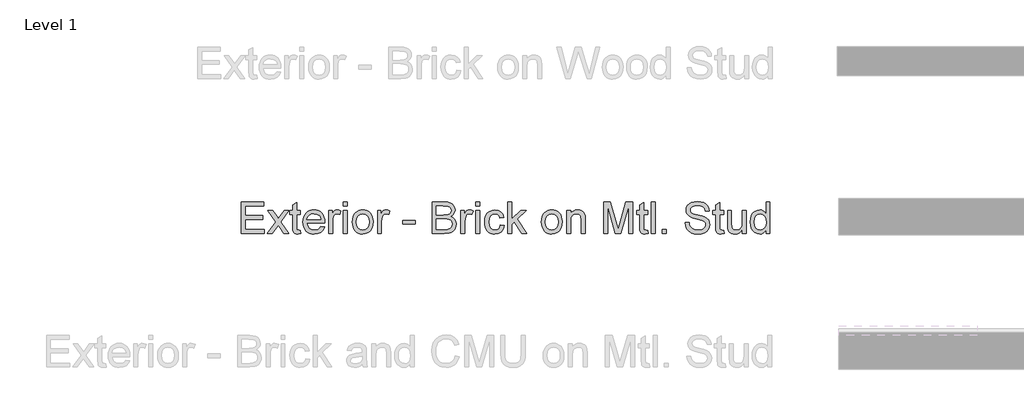
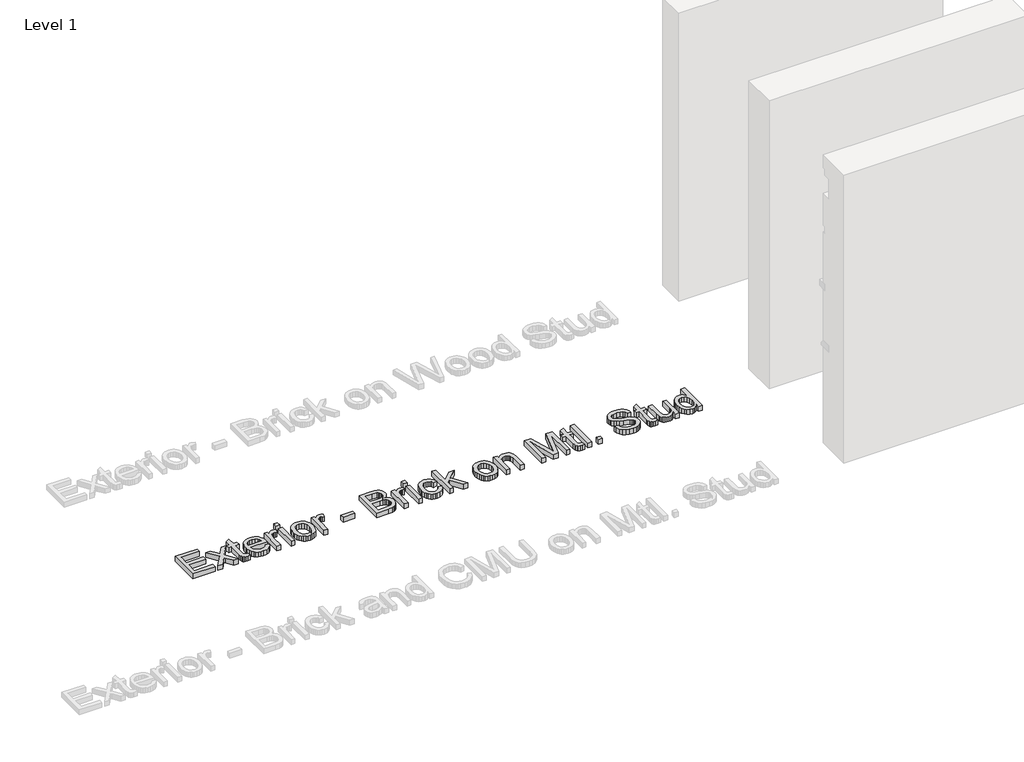
# One storey, part 27 of 42: 1 proxy.
"""IFC4 building model written with IfcOpenShell, lengths in millimetres."""

from ifc_helpers import new_model, si_unit, origin, origin_with_axes, place, context, project, spatial, polyline, outline, extrude, element, save

model = new_model("IFC4")

# Units and contexts
model_context = context("Model", 3, world=origin())
ifc_project = project(units=[si_unit("LENGTHUNIT", "METRE", prefix="MILLI")], contexts=[model_context])

# Site, building, storey
site = spatial("IfcSite", under=ifc_project)
building = spatial("IfcBuilding", under=site)
storey = spatial("IfcBuildingStorey", under=building, Name="Level 1", Elevation=0.0)

# Proxy
placement = place(None, origin())
element("IfcBuildingElementProxy", 1, Name="8\" Arial", ObjectType="8\" Arial", at=placement, inside=storey, context=model_context, shape_type="SweptSolid", body=[
    extrude(outline(polyline([(-5074.4671902, 11235.919571), (-5074.4671902, 11540.4866651), (-4855.5595914, 11540.4866651), (-4855.5595914, 11502.4157783), (-5036.3963035, 11502.4157783), (-5036.3963035, 11411.9974223), (-4865.0773131, 11411.9974223), (-4865.0773131, 11373.9265355), (-5036.3963035, 11373.9265355), (-5036.3963035, 11273.9904578), (-4850.8007305, 11273.9904578), (-4850.8007305, 11235.919571), (-5074.4671902, 11235.919571)])), origin_with_axes(), (0.0, 0.0, 1.0), 50.8),
    extrude(outline(polyline([(-4822.2475655, 11235.919571), (-4740.9007879, 11348.3476585), (-4817.4887046, 11459.5860307), (-4771.684669, 11459.5860307), (-4734.7291402, 11406.0488462), (-4717.4782697, 11380.767398), (-4702.5324723, 11401.4386998), (-4660.4462967, 11459.5860307), (-4614.6422611, 11459.5860307), (-4695.0967523, 11348.3476585), (-4617.6165491, 11235.919571), (-4663.4205848, 11235.919571), (-4710.0425496, 11303.5102665), (-4718.5936277, 11315.8535618), (-4776.4435298, 11235.919571), (-4822.2475655, 11235.919571)])), origin_with_axes(), (0.0, 0.0, 1.0), 50.8),
    extrude(outline(polyline([(-4503.4038889, 11267.6700957), (-4498.645028, 11234.804213), (-4527.1238359, 11231.1607102), (-4545.397118, 11232.7408007), (-4559.023075, 11237.4810723), (-4568.6523325, 11244.7866672), (-4574.9355159, 11254.062728), (-4578.3931258, 11269.9937583), (-4579.5456624, 11297.2642616), (-4579.5456624, 11421.515144), (-4608.0988274, 11421.515144), (-4608.0988274, 11459.5860307), (-4579.5456624, 11459.5860307), (-4579.5456624, 11513.9411445), (-4541.4747756, 11536.3226619), (-4541.4747756, 11459.5860307), (-4503.4038889, 11459.5860307), (-4503.4038889, 11421.515144), (-4541.4747756, 11421.515144), (-4541.4747756, 11298.3796196), (-4539.4671312, 11278.7493186), (-4532.9608761, 11271.7969204), (-4519.9855446, 11269.231597), (-4503.4038889, 11267.6700957)])), origin_with_axes(), (0.0, 0.0, 1.0), 50.8),
    extrude(outline(polyline([(-4308.7367374, 11302.5436229), (-4271.4094227, 11297.784762), (-4284.8587814, 11269.6591509), (-4306.3201284, 11248.6346524), (-4335.310142, 11235.5291957), (-4371.3455004, 11231.1607102), (-4394.9678536, 11233.0452005), (-4416.0155887, 11238.6986714), (-4434.4887058, 11248.1211229), (-4450.3872048, 11261.3125551), (-4463.171996, 11277.9058291), (-4472.3039897, 11297.5338065), (-4477.7831859, 11320.196487), (-4479.6095846, 11345.8938709), (-4477.7645966, 11372.4626281), (-4472.2296325, 11395.880499), (-4463.0046923, 11416.1474836), (-4450.089776, 11433.2635817), (-4434.2331029, 11446.8616548), (-4416.1828924, 11456.5745641), (-4395.9391445, 11462.4023097), (-4373.5018592, 11464.3448916), (-4351.787233, 11462.406957), (-4332.149961, 11456.5931534), (-4314.5900433, 11446.9034807), (-4299.1074799, 11433.3379389), (-4286.4690795, 11416.2590194), (-4277.4416506, 11396.0292134), (-4272.0251932, 11372.6485212), (-4270.2197075, 11346.1169425), (-4270.4427791, 11335.8556488), (-4441.5386979, 11335.8556488), (-4434.948791, 11307.3582516), (-4419.6405023, 11286.4081103), (-4397.547119, 11273.5257253), (-4370.6019284, 11269.231597), (-4350.3395912, 11271.2206521), (-4333.2746137, 11277.1878174), (-4319.4069957, 11287.504879), (-4308.7367374, 11302.5436229)]), holes=[polyline([(-4441.5386979, 11373.9265355), (-4308.2905942, 11373.9265355), (-4313.4398304, 11394.0401583), (-4323.5338204, 11408.4282767), (-4345.7294448, 11421.8125728), (-4373.6505736, 11426.2740048), (-4399.3131025, 11422.7141538), (-4420.5327887, 11412.0346009), (-4435.2833984, 11395.3878826), (-4441.5386979, 11373.9265355)])]), origin_with_axes(), (0.0, 0.0, 1.0), 50.8),
    extrude(outline(polyline([(-4232.1488207, 11235.919571), (-4232.1488207, 11459.5860307), (-4198.8367948, 11459.5860307), (-4198.8367948, 11426.4970764), (-4186.5306781, 11445.6812342), (-4175.191205, 11456.9835287), (-4163.8145533, 11462.5045509), (-4151.3969007, 11464.3448916), (-4132.4358146, 11461.4077822), (-4113.1772996, 11452.5964539), (-4125.8923809, 11418.4664988), (-4139.276677, 11424.3221283), (-4152.6609732, 11426.2740048), (-4164.0283302, 11424.3964855), (-4174.1873828, 11418.7639276), (-4182.3945588, 11409.8038849), (-4187.9062863, 11397.9439114), (-4192.535022, 11376.677752), (-4194.0779339, 11353.4783053), (-4194.0779339, 11235.919571), (-4232.1488207, 11235.919571)])), origin_with_axes(), (0.0, 0.0, 1.0), 50.8),
    extrude(outline(polyline([(-4089.3829954, 11502.4157783), (-4089.3829954, 11540.4866651), (-4051.3121086, 11540.4866651), (-4051.3121086, 11502.4157783), (-4089.3829954, 11502.4157783)])), origin_with_axes(), (0.0, 0.0, 1.0), 50.8),
    extrude(outline(polyline([(-4089.3829954, 11235.919571), (-4089.3829954, 11459.5860307), (-4051.3121086, 11459.5860307), (-4051.3121086, 11235.919571), (-4089.3829954, 11235.919571)])), origin_with_axes(), (0.0, 0.0, 1.0), 50.8),
    extrude(outline(polyline([(-4003.7235002, 11347.7528009), (-4001.6647352, 11376.7195779), (-3995.4884402, 11401.6803607), (-3985.1946152, 11422.6351493), (-3970.7832602, 11439.5839438), (-3956.2743115, 11450.4168584), (-3940.2596294, 11458.1546546), (-3922.7392139, 11462.7973323), (-3903.7130652, 11464.3448916), (-3882.7094797, 11462.4604013), (-3863.7181859, 11456.8069304), (-3846.7391838, 11447.3844788), (-3831.7724735, 11434.1930467), (-3819.5569797, 11417.6787772), (-3810.8316269, 11398.2878134), (-3805.5964152, 11376.0201555), (-3803.8513447, 11350.8758033), (-3806.9371685, 11312.4145413), (-3816.19464, 11283.1363935), (-3831.3542143, 11261.2103139), (-3852.1463465, 11244.8052565), (-3876.8422318, 11234.5718468), (-3903.7130652, 11231.1607102), (-3925.0233742, 11233.0382295), (-3944.1912663, 11238.6707875), (-3961.2167416, 11248.0583841), (-3976.0998001, 11261.2010193), (-3988.1851689, 11277.8756215), (-3996.8175751, 11297.8591192), (-4001.9970189, 11321.1515123), (-4003.7235002, 11347.7528009)]), holes=[polyline([(-3965.6526134, 11347.8271581), (-3961.2469493, 11313.3718902), (-3948.0299568, 11288.8247193), (-3928.1394056, 11274.1298775), (-3903.7130652, 11269.231597), (-3879.3982606, 11274.1577615), (-3859.544888, 11288.9362551), (-3846.3278956, 11313.8087388), (-3841.9222314, 11349.0168733), (-3846.3557795, 11382.468319), (-3859.6564238, 11406.6808824), (-3879.5376803, 11421.3757242), (-3903.7130652, 11426.2740048), (-3928.1394056, 11421.3943135), (-3948.0299568, 11406.7552396), (-3961.2469493, 11382.2638367), (-3965.6526134, 11347.8271581)])]), origin_with_axes(), (0.0, 0.0, 1.0), 50.8),
    extrude(outline(polyline([(-3761.0215971, 11235.919571), (-3761.0215971, 11459.5860307), (-3727.7095712, 11459.5860307), (-3727.7095712, 11426.4970764), (-3715.4034544, 11445.6812342), (-3704.0639813, 11456.9835287), (-3692.6873296, 11462.5045509), (-3680.2696771, 11464.3448916), (-3661.3085909, 11461.4077822), (-3642.0500759, 11452.5964539), (-3654.7651573, 11418.4664988), (-3668.1494534, 11424.3221283), (-3681.5337495, 11426.2740048), (-3692.9011066, 11424.3964855), (-3703.0601591, 11418.7639276), (-3711.2673352, 11409.8038849), (-3716.7790627, 11397.9439114), (-3721.4077984, 11376.677752), (-3722.9507103, 11353.4783053), (-3722.9507103, 11235.919571), (-3761.0215971, 11235.919571)])), origin_with_axes(), (0.0, 0.0, 1.0), 50.8),
    extrude(outline(polyline([(-3518.319694, 11326.3379271), (-3518.319694, 11364.4088138), (-3399.3481729, 11364.4088138), (-3399.3481729, 11326.3379271), (-3518.319694, 11326.3379271)])), origin_with_axes(), (0.0, 0.0, 1.0), 50.8),
    extrude(outline(polyline([(-3232.7880433, 11235.919571), (-3232.7880433, 11540.4866651), (-3116.5677386, 11540.4866651), (-3084.6034369, 11538.2466544), (-3059.6473015, 11531.5266224), (-3040.5189116, 11520.1592654), (-3026.0378467, 11503.9772796), (-3016.919795, 11484.9418362), (-3013.8804444, 11465.0141064), (-3016.4364732, 11446.6757618), (-3024.1045595, 11429.4341859), (-3036.9404713, 11414.3489688), (-3054.9999764, 11402.4797006), (-3033.4270936, 11391.2145847), (-3017.4867687, 11374.0752499), (-3007.6437342, 11352.1956436), (-3004.3627227, 11326.7097131), (-3006.6027334, 11305.4714376), (-3013.3227654, 11285.7760741), (-3023.3516929, 11269.0271146), (-3035.5183898, 11256.6280514), (-3050.4177139, 11247.6494194), (-3068.6445227, 11241.1617537), (-3117.460025, 11235.919571), (-3232.7880433, 11235.919571)]), holes=[polyline([(-3194.7171565, 11416.7562831), (-3125.1931739, 11416.7562831), (-3084.5941423, 11420.028), (-3070.3826223, 11425.6698526), (-3060.1678019, 11434.1186895), (-3054.0054489, 11445.2443857), (-3051.9513312, 11458.9168159), (-3053.8660291, 11472.1895763), (-3059.6101229, 11483.752121), (-3068.9233623, 11492.7772262), (-3081.5454971, 11498.4376681), (-3130.4725351, 11502.4157783), (-3194.7171565, 11502.4157783), (-3194.7171565, 11416.7562831)]), polyline([(-3194.7171565, 11273.9904578), (-3116.6420958, 11273.9904578), (-3088.3863595, 11275.4776018), (-3064.4805195, 11283.7684297), (-3048.6424358, 11300.6846928), (-3043.9858161, 11312.6376129), (-3042.4336095, 11326.3379271), (-3044.2553609, 11342.250368), (-3049.7206152, 11355.932093), (-3059.2662208, 11366.6302352), (-3073.3290264, 11373.5919281), (-3093.2474615, 11377.4120293), (-3120.3599558, 11378.6853964), (-3194.7171565, 11378.6853964), (-3194.7171565, 11273.9904578)])]), origin_with_axes(), (0.0, 0.0, 1.0), 50.8),
    extrude(outline(polyline([(-2956.7741143, 11235.919571), (-2956.7741143, 11459.5860307), (-2923.4620884, 11459.5860307), (-2923.4620884, 11426.4970764), (-2911.1559717, 11445.6812342), (-2899.8164986, 11456.9835287), (-2888.4398469, 11462.5045509), (-2876.0221943, 11464.3448916), (-2857.0611082, 11461.4077822), (-2837.8025932, 11452.5964539), (-2850.5176745, 11418.4664988), (-2863.9019706, 11424.3221283), (-2877.2862667, 11426.2740048), (-2888.6536238, 11424.3964855), (-2898.8126763, 11418.7639276), (-2907.0198524, 11409.8038849), (-2912.5315799, 11397.9439114), (-2917.1603156, 11376.677752), (-2918.7032275, 11353.4783053), (-2918.7032275, 11235.919571), (-2956.7741143, 11235.919571)])), origin_with_axes(), (0.0, 0.0, 1.0), 50.8),
    extrude(outline(polyline([(-2814.008289, 11235.919571), (-2814.008289, 11459.5860307), (-2775.9374022, 11459.5860307), (-2775.9374022, 11235.919571), (-2814.008289, 11235.919571)])), origin_with_axes(), (0.0, 0.0, 1.0), 50.8),
    extrude(outline(polyline([(-2814.008289, 11502.4157783), (-2814.008289, 11540.4866651), (-2775.9374022, 11540.4866651), (-2775.9374022, 11502.4157783), (-2814.008289, 11502.4157783)])), origin_with_axes(), (0.0, 0.0, 1.0), 50.8),
    extrude(outline(polyline([(-2576.0652467, 11316.8202054), (-2537.99436, 11312.0613446), (-2548.6088504, 11278.2009343), (-2568.5551694, 11252.6127626), (-2595.9557979, 11236.5237233), (-2628.9332164, 11231.1607102), (-2650.2853513, 11233.0312585), (-2669.4300068, 11238.6429035), (-2686.367183, 11247.9956452), (-2701.0968797, 11261.0894835), (-2713.0195921, 11277.6781102), (-2721.5358152, 11297.5152172), (-2726.6455491, 11320.6008043), (-2728.3487937, 11346.9348717), (-2725.4395683, 11380.8138713), (-2716.7118918, 11410.1756709), (-2702.0263447, 11433.8863233), (-2681.2435071, 11450.8118811), (-2656.3803181, 11460.961639), (-2629.4537168, 11464.3448916), (-2597.2849329, 11459.6975665), (-2571.5666361, 11445.7555914), (-2553.1167556, 11423.2625382), (-2542.7532208, 11392.9619789), (-2580.8241076, 11388.2031181), (-2587.7300326, 11404.8126578), (-2598.4839427, 11416.7191045), (-2612.4909804, 11423.8852798), (-2629.156288, 11426.2740048), (-2653.7592268, 11421.5709119), (-2673.2872866, 11407.4616331), (-2686.0302519, 11383.184007), (-2690.277907, 11347.9758725), (-2686.1231984, 11312.2937108), (-2673.6590726, 11287.9324329), (-2654.4842095, 11273.9068059), (-2630.1972888, 11269.231597), (-2610.483336, 11272.1501171), (-2594.3199395, 11280.9056775), (-2582.5622071, 11295.7213497), (-2576.0652467, 11316.8202054)])), origin_with_axes(), (0.0, 0.0, 1.0), 50.8),
    extrude(outline(polyline([(-2504.682334, 11235.919571), (-2504.682334, 11540.4866651), (-2466.6114473, 11540.4866651), (-2466.6114473, 11376.8264664), (-2381.2493809, 11459.5860307), (-2328.6044828, 11459.5860307), (-2415.00755, 11375.7854656), (-2323.8456219, 11235.919571), (-2368.311228, 11235.919571), (-2442.2966427, 11349.3143021), (-2466.6114473, 11325.7430695), (-2466.6114473, 11235.919571), (-2504.682334, 11235.919571)])), origin_with_axes(), (0.0, 0.0, 1.0), 50.8),
    extrude(outline(polyline([(-2181.0797966, 11347.7528009), (-2179.0210316, 11376.7195779), (-2172.8447366, 11401.6803607), (-2162.5509116, 11422.6351493), (-2148.1395567, 11439.5839438), (-2133.6306079, 11450.4168584), (-2117.6159258, 11458.1546546), (-2100.0955104, 11462.7973323), (-2081.0693616, 11464.3448916), (-2060.0657761, 11462.4604013), (-2041.0744823, 11456.8069304), (-2024.0954803, 11447.3844788), (-2009.12877, 11434.1930467), (-1996.9132761, 11417.6787772), (-1988.1879233, 11398.2878134), (-1982.9527117, 11376.0201555), (-1981.2076411, 11350.8758033), (-1984.2934649, 11312.4145413), (-1993.5509364, 11283.1363935), (-2008.7105107, 11261.2103139), (-2029.502643, 11244.8052565), (-2054.1985282, 11234.5718468), (-2081.0693616, 11231.1607102), (-2102.3796706, 11233.0382295), (-2121.5475628, 11238.6707875), (-2138.5730381, 11248.0583841), (-2153.4560965, 11261.2010193), (-2165.5414653, 11277.8756215), (-2174.1738716, 11297.8591192), (-2179.3533153, 11321.1515123), (-2181.0797966, 11347.7528009)]), holes=[polyline([(-2143.0089098, 11347.8271581), (-2138.6032457, 11313.3718902), (-2125.3862533, 11288.8247193), (-2105.4957021, 11274.1298775), (-2081.0693616, 11269.231597), (-2056.754557, 11274.1577615), (-2036.9011844, 11288.9362551), (-2023.684192, 11313.8087388), (-2019.2785279, 11349.0168733), (-2023.712076, 11382.468319), (-2037.0127202, 11406.6808824), (-2056.8939768, 11421.3757242), (-2081.0693616, 11426.2740048), (-2105.4957021, 11421.3943135), (-2125.3862533, 11406.7552396), (-2138.6032457, 11382.2638367), (-2143.0089098, 11347.8271581)])]), origin_with_axes(), (0.0, 0.0, 1.0), 50.8),
    extrude(outline(polyline([(-1938.3778935, 11235.919571), (-1938.3778935, 11459.5860307), (-1900.3070067, 11459.5860307), (-1900.3070067, 11428.3560064), (-1887.0807197, 11444.1011437), (-1871.1961627, 11455.3476703), (-1852.6533357, 11462.0955863), (-1831.4522389, 11464.3448916), (-1812.6863404, 11462.5324348), (-1795.5005324, 11457.0950645), (-1781.1681819, 11448.7112901), (-1770.9626561, 11438.0596211), (-1759.5488258, 11410.0641351), (-1757.5411814, 11373.2573207), (-1757.5411814, 11235.919571), (-1795.6120682, 11235.919571), (-1795.6120682, 11368.1266739), (-1799.999143, 11401.8104858), (-1806.0685495, 11411.8394132), (-1815.5026193, 11419.6190354), (-1827.5949591, 11424.6102625), (-1841.6391754, 11426.2740048), (-1863.937041, 11422.5375555), (-1882.9446004, 11411.3282075), (-1890.5406532, 11402.1776245), (-1895.9664052, 11389.6716728), (-1900.3070067, 11354.5936634), (-1900.3070067, 11235.919571), (-1938.3778935, 11235.919571)])), origin_with_axes(), (0.0, 0.0, 1.0), 50.8),
    extrude(outline(polyline([(-1581.4633301, 11235.919571), (-1581.4633301, 11540.4866651), (-1515.9546363, 11540.4866651), (-1453.6433021, 11325.8174267), (-1441.0769352, 11280.9800347), (-1427.4695675, 11329.5352867), (-1366.1992341, 11540.4866651), (-1300.6905403, 11540.4866651), (-1300.6905403, 11235.919571), (-1338.7614271, 11235.919571), (-1338.7614271, 11502.4157783), (-1415.2749866, 11235.919571), (-1466.8788839, 11235.919571), (-1543.3924434, 11502.4157783), (-1543.3924434, 11235.919571), (-1581.4633301, 11235.919571)])), origin_with_axes(), (0.0, 0.0, 1.0), 50.8),
    extrude(outline(polyline([(-1157.924715, 11267.6700957), (-1153.1658541, 11234.804213), (-1181.644662, 11231.1607102), (-1199.917944, 11232.7408007), (-1213.5439011, 11237.4810723), (-1223.1731586, 11244.7866672), (-1229.456342, 11254.062728), (-1232.9139519, 11269.9937583), (-1234.0664885, 11297.2642616), (-1234.0664885, 11421.515144), (-1262.6196535, 11421.515144), (-1262.6196535, 11459.5860307), (-1234.0664885, 11459.5860307), (-1234.0664885, 11513.9411445), (-1195.9956017, 11536.3226619), (-1195.9956017, 11459.5860307), (-1157.924715, 11459.5860307), (-1157.924715, 11421.515144), (-1195.9956017, 11421.515144), (-1195.9956017, 11298.3796196), (-1193.9879573, 11278.7493186), (-1187.4817022, 11271.7969204), (-1174.5063707, 11269.231597), (-1157.924715, 11267.6700957)])), origin_with_axes(), (0.0, 0.0, 1.0), 50.8),
    extrude(outline(polyline([(-1119.8538282, 11235.919571), (-1119.8538282, 11540.4866651), (-1081.7829414, 11540.4866651), (-1081.7829414, 11235.919571), (-1119.8538282, 11235.919571)])), origin_with_axes(), (0.0, 0.0, 1.0), 50.8),
    extrude(outline(polyline([(-1015.1588896, 11235.919571), (-1015.1588896, 11273.9904578), (-977.0880029, 11273.9904578), (-977.0880029, 11235.919571), (-1015.1588896, 11235.919571)])), origin_with_axes(), (0.0, 0.0, 1.0), 50.8),
    extrude(outline(polyline([(-796.2512907, 11340.6145096), (-758.180404, 11340.6145096), (-753.8119184, 11319.48777), (-745.9114659, 11302.5064443), (-733.5867599, 11289.0292016), (-715.945514, 11278.4147112), (-694.3819258, 11271.5273755), (-670.2901928, 11269.231597), (-649.0798013, 11270.9696965), (-630.5090904, 11276.1839952), (-615.4610519, 11284.4376445), (-604.8186775, 11295.2937958), (-598.4890208, 11307.7579216), (-596.3791353, 11320.8354942), (-597.9592258, 11333.5784595), (-602.6994973, 11344.5926199), (-612.3287548, 11353.9895111), (-628.5758032, 11361.880669), (-684.0090963, 11376.4175018), (-720.3976514, 11386.0374646), (-743.6807499, 11395.1926949), (-762.6325414, 11408.0007228), (-776.0633108, 11423.5227884), (-784.0660045, 11441.4242845), (-786.7335691, 11461.3706036), (-783.4339683, 11483.6684691), (-773.5351659, 11504.4606014), (-757.2974122, 11522.0832579), (-734.9809574, 11534.8726965), (-708.1937758, 11542.6523186), (-678.543842, 11545.245526), (-646.4215313, 11542.5314881), (-618.3145095, 11534.3893746), (-595.2265987, 11520.9864892), (-578.1616211, 11502.4901355), (-567.3612377, 11480.0528502), (-563.0671094, 11454.8271699), (-601.1379961, 11454.8271699), (-608.127573, 11477.5432947), (-622.7015843, 11493.9390575), (-645.473477, 11503.8657438), (-677.056698, 11507.1746392), (-709.383491, 11503.9029224), (-731.5605261, 11494.0877719), (-744.3871433, 11479.6438856), (-748.6626823, 11462.4859616), (-745.6326264, 11447.8561823), (-736.5424586, 11436.0891553), (-715.0532276, 11425.5676114), (-674.3798388, 11414.8229959), (-632.405199, 11404.6174701), (-607.012215, 11395.7131953), (-585.309207, 11381.9013453), (-570.168222, 11364.8549571), (-561.2732419, 11344.7599236), (-558.3082485, 11321.8021378), (-561.7193851, 11298.3331464), (-571.9527948, 11276.2583524), (-588.5902185, 11257.2600876), (-611.2133968, 11243.0206837), (-638.4188376, 11234.1257036), (-668.8030487, 11231.1607102), (-706.1024795, 11234.3580698), (-736.8027088, 11243.9501487), (-761.2569332, 11259.9741255), (-779.8183494, 11282.4671787), (-791.7340908, 11309.8678071), (-796.2512907, 11340.6145096)])), origin_with_axes(), (0.0, 0.0, 1.0), 50.8),
    extrude(outline(polyline([(-425.0601449, 11267.6700957), (-420.301284, 11234.804213), (-448.7800919, 11231.1607102), (-467.0533739, 11232.7408007), (-480.679331, 11237.4810723), (-490.3085885, 11244.7866672), (-496.5917719, 11254.062728), (-500.0493818, 11269.9937583), (-501.2019184, 11297.2642616), (-501.2019184, 11421.515144), (-529.7550834, 11421.515144), (-529.7550834, 11459.5860307), (-501.2019184, 11459.5860307), (-501.2019184, 11513.9411445), (-463.1310316, 11536.3226619), (-463.1310316, 11459.5860307), (-425.0601449, 11459.5860307), (-425.0601449, 11421.515144), (-463.1310316, 11421.515144), (-463.1310316, 11298.3796196), (-461.1233872, 11278.7493186), (-454.6171321, 11271.7969204), (-441.6418006, 11269.231597), (-425.0601449, 11267.6700957)])), origin_with_axes(), (0.0, 0.0, 1.0), 50.8),
    extrude(outline(polyline([(-244.2234327, 11235.919571), (-244.2234327, 11274.3622438), (-257.9981042, 11255.4615728), (-274.0406702, 11241.9610936), (-292.3511309, 11233.860806), (-312.9294862, 11231.1607102), (-331.4723131, 11233.0568188), (-348.7324783, 11238.7451447), (-363.2135432, 11247.2962227), (-373.419069, 11257.780588), (-380.2878154, 11270.5142587), (-384.7585421, 11285.8132527), (-386.9892581, 11321.2072802), (-386.9892581, 11459.5860307), (-348.9183713, 11459.5860307), (-348.9183713, 11339.1273656), (-346.6132981, 11300.3129068), (-341.064392, 11287.3654593), (-331.555965, 11277.5224248), (-318.7200532, 11271.3043039), (-303.1886929, 11269.231597), (-286.7650462, 11271.3507772), (-271.4009896, 11277.7083178), (-258.7323815, 11287.718656), (-250.3950804, 11300.7962286), (-245.7663447, 11318.7070194), (-244.2234327, 11343.2170116), (-244.2234327, 11459.5860307), (-206.152546, 11459.5860307), (-206.152546, 11235.919571), (-244.2234327, 11235.919571)])), origin_with_axes(), (0.0, 0.0, 1.0), 50.8),
    extrude(outline(polyline([(-15.7981122, 11235.919571), (-15.7981122, 11271.834099), (-27.1887059, 11254.0394914), (-40.9866139, 11241.3290574), (-57.1918364, 11233.702797), (-75.8043732, 11231.1607102), (-100.4166066, 11234.8413916), (-122.9468384, 11245.8834359), (-142.0194604, 11263.5153871), (-156.2588643, 11286.9657893), (-165.1259605, 11315.2865881), (-168.0816592, 11347.5297293), (-165.3583268, 11379.3732005), (-157.1883293, 11408.1308479), (-143.5809616, 11432.166813), (-124.5455182, 11449.8452375), (-101.52267, 11460.7199781), (-75.9530876, 11464.3448916), (-57.3266088, 11461.7516842), (-40.8564888, 11453.9720621), (-26.8959244, 11442.047026), (-15.7981122, 11427.0175768), (-15.7981122, 11540.4866651), (22.2727746, 11540.4866651), (22.2727746, 11235.919571), (-15.7981122, 11235.919571)]), holes=[polyline([(-130.0107725, 11347.6784437), (-125.7166441, 11313.2417651), (-112.8342591, 11288.7503621), (-94.1148338, 11274.1112882), (-72.3095847, 11269.231597), (-50.5136303, 11273.8882166), (-32.2682322, 11287.8580757), (-19.9156422, 11311.4014244), (-15.7981122, 11344.7785129), (-19.9899994, 11381.2693091), (-32.565661, 11406.5693466), (-51.2757916, 11421.3478403), (-73.8710859, 11426.2740048), (-95.8994067, 11421.5430279), (-113.9496171, 11407.3500973), (-125.9954836, 11382.9702301), (-130.0107725, 11347.6784437)])]), origin_with_axes(), (0.0, 0.0, 1.0), 50.8),
])

save(model, "model.ifc")

# Revit data of these elements
# Element 1 (IfcBuildingElementProxy, "8\" Arial")
#   Phase Created = New Construction
